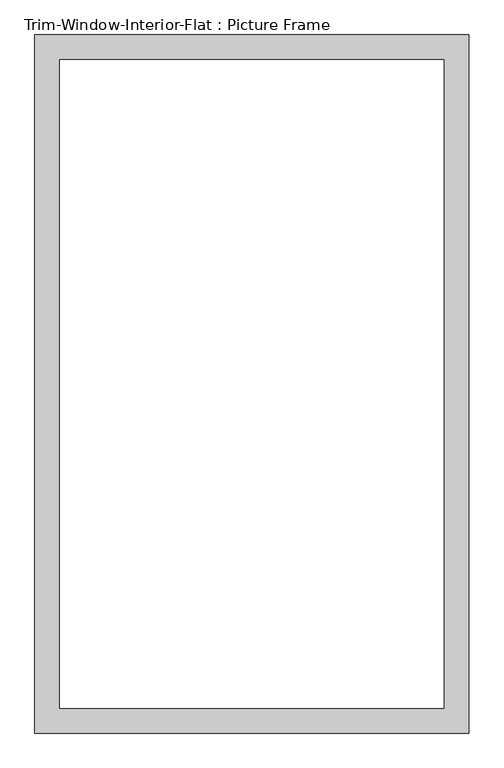
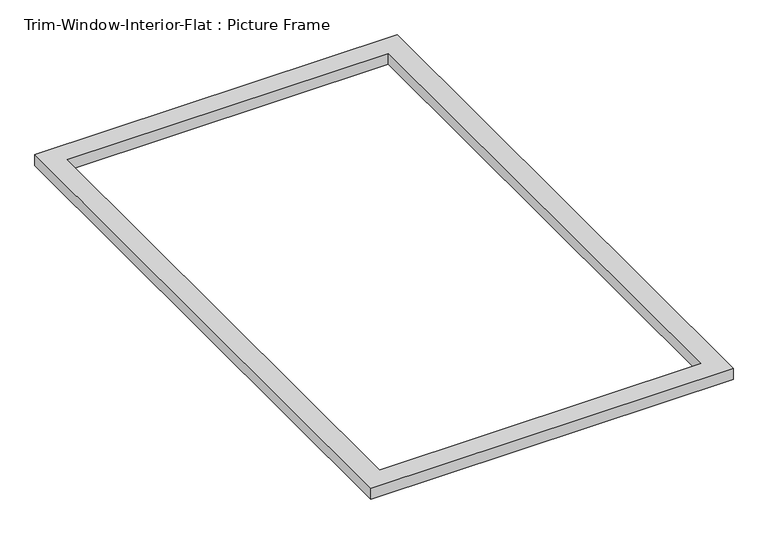
"""IFC4 building model written with IfcOpenShell, lengths in millimetres: proxy geometry, Trim-Window-Interior-Flat : Picture Frame."""

import ifcopenshell
import ifcopenshell.guid

model = None  # the IFC model being written
_history = None  # IfcOwnerHistory: only IFC2X3 demands one
_inside = {}  # id of a spatial element -> (the spatial element, [elements in it])
_under = {}  # id of a project, library or spatial element -> (it, [spatial elements below it])
_declared = {}  # id of a project -> (the project, [libraries it declares])
_typed = {}  # id of a type object -> (the type object, [elements of that type])
_made_of = {}  # id of a material, layer set ... -> (it, [elements and type objects made of it])


def new_model(schema):
    """Start an empty IFC model of exactly this schema.

    Asked for "IFC4X3", IfcOpenShell would pick the latest addendum, in which some entities
    have other attributes; the version numbers below select the first issue.
    IFC2X3 requires an IfcOwnerHistory on every rooted entity: one is made here for all.
    """
    global model, _history
    if schema == "IFC4X3":
        model = ifcopenshell.file(schema_version=(4, 3, 0, 0))
    else:
        model = ifcopenshell.file(schema=schema)
    _inside.clear()
    _under.clear()
    _declared.clear()
    _typed.clear()
    _made_of.clear()
    _history = None
    if model.schema == "IFC2X3":
        org = make("IfcOrganization", Name="unknown")
        user = make(
            "IfcPersonAndOrganization",
            ThePerson=make("IfcPerson", FamilyName="unknown"),
            TheOrganization=org,
        )
        app = make(
            "IfcApplication",
            ApplicationDeveloper=org,
            Version="unknown",
            ApplicationFullName="unknown",
            ApplicationIdentifier="unknown",
        )
        _history = make(
            "IfcOwnerHistory",
            OwningUser=user,
            OwningApplication=app,
            ChangeAction="ADDED",
            CreationDate=0,
        )
    return model


def make(cls, **values):
    """One entity of the class cls with the attributes given. An attribute that is None is left unset."""
    return model.create_entity(
        cls, **{name: value for name, value in values.items() if value is not None}
    )


def rooted(cls, **values):
    """An entity with a GlobalId (a new one), such as an element, a storey or a relation."""
    return make(cls, GlobalId=ifcopenshell.guid.new(), OwnerHistory=_history, **values)


def si_unit(unit_type, name, prefix=None):
    """IfcSIUnit, for example si_unit("LENGTHUNIT", "METRE", prefix="MILLI")."""
    return make("IfcSIUnit", UnitType=unit_type, Prefix=prefix, Name=name)


def assignment(units):
    """IfcUnitAssignment: the units of a project."""
    return None if units is None else make("IfcUnitAssignment", Units=units)


def point(xyz):
    """IfcCartesianPoint."""
    return None if xyz is None else make("IfcCartesianPoint", Coordinates=xyz)


def direction(xyz):
    """IfcDirection."""
    return None if xyz is None else make("IfcDirection", DirectionRatios=xyz)


def frame(location, z_axis=None, x_axis=None):
    """IfcAxis2Placement3D, a coordinate frame: its origin and axes. An axis left out is left unset."""
    return make(
        "IfcAxis2Placement3D",
        Location=point(location),
        Axis=direction(z_axis),
        RefDirection=direction(x_axis),
    )


def origin():
    """The frame at (0, 0, 0) with its axes left unset."""
    return frame((0.0, 0.0, 0.0))


def origin_with_axes():
    """The frame at (0, 0, 0) with the z axis (0, 0, 1) and the x axis (1, 0, 0) written out."""
    return frame((0.0, 0.0, 0.0), z_axis=(0.0, 0.0, 1.0), x_axis=(1.0, 0.0, 0.0))


def place(relative_to, where):
    """IfcLocalPlacement: puts the frame where relative to a parent placement (None: the world)."""
    return make(
        "IfcLocalPlacement", PlacementRelTo=relative_to, RelativePlacement=where
    )


def context(
    kind, dimensions, precision=None, world=None, true_north=None, identifier=None
):
    """IfcGeometricRepresentationContext, for example the 3D "Model" context."""
    return make(
        "IfcGeometricRepresentationContext",
        ContextIdentifier=identifier,
        ContextType=kind,
        CoordinateSpaceDimension=dimensions,
        Precision=precision,
        WorldCoordinateSystem=world,
        TrueNorth=true_north,
    )


def project(units=None, contexts=None):
    """IfcProject with its units and contexts."""
    return rooted(
        "IfcProject",
        Name="project",
        RepresentationContexts=contexts,
        UnitsInContext=assignment(units),
    )


def spatial(cls, under=None, at=None, **own):
    """A site, building, storey or space (cls), placed at a placement, below another one or the project."""
    s = rooted(cls, ObjectPlacement=at, **own)
    if under is not None:
        _under.setdefault(under.id(), (under, []))[1].append(s)
    return s


def polyline(points):
    """IfcPolyline through the points."""
    return make("IfcPolyline", Points=[point(p) for p in points])


def outline(outer, holes=None, kind="AREA"):
    """IfcArbitraryClosedProfileDef: a profile drawn as a closed curve; with holes, ...WithVoids."""
    if holes is None:
        return make("IfcArbitraryClosedProfileDef", ProfileType=kind, OuterCurve=outer)
    return make(
        "IfcArbitraryProfileDefWithVoids",
        ProfileType=kind,
        OuterCurve=outer,
        InnerCurves=holes,
    )


def extrude(swept, where, along, depth):
    """IfcExtrudedAreaSolid: the profile swept, set in the frame where, extruded along a direction by depth."""
    return make(
        "IfcExtrudedAreaSolid",
        SweptArea=swept,
        Position=where,
        ExtrudedDirection=direction(along),
        Depth=depth,
    )


def shape(context_of_items, identifier, shape_type, items):
    """IfcShapeRepresentation: the items that make up one representation, for example the "Body"."""
    return make(
        "IfcShapeRepresentation",
        ContextOfItems=context_of_items,
        RepresentationIdentifier=identifier,
        RepresentationType=shape_type,
        Items=items,
    )


def source(mapping_origin, context_of_items, identifier, shape_type, items):
    """IfcRepresentationMap: a shape defined once, which mapped items show again and again."""
    return make(
        "IfcRepresentationMap",
        MappingOrigin=mapping_origin,
        MappedRepresentation=shape(context_of_items, identifier, shape_type, items),
    )


def transform(
    local_origin,
    x_axis=None,
    y_axis=None,
    z_axis=None,
    scale=None,
    scale2=None,
    scale3=None,
    uniform=True,
):
    """IfcCartesianTransformationOperator3D, or its non-uniform kind. x_axis, y_axis, z_axis: its Axis1, 2, 3."""
    if uniform:
        return make(
            "IfcCartesianTransformationOperator3D",
            Axis1=direction(x_axis),
            Axis2=direction(y_axis),
            LocalOrigin=point(local_origin),
            Scale=scale,
            Axis3=direction(z_axis),
        )
    return make(
        "IfcCartesianTransformationOperator3DnonUniform",
        Axis1=direction(x_axis),
        Axis2=direction(y_axis),
        LocalOrigin=point(local_origin),
        Scale=scale,
        Axis3=direction(z_axis),
        Scale2=scale2,
        Scale3=scale3,
    )


def mapped(mapping_source, mapping_target):
    """IfcMappedItem: shows the shape of a source again, moved by a transform."""
    return make(
        "IfcMappedItem", MappingSource=mapping_source, MappingTarget=mapping_target
    )


def made_of(thing, what):
    """Note that an element or type object is made of a material, layer set ...; save() writes the relation."""
    if what is not None:
        _made_of.setdefault(what.id(), (what, []))[1].append(thing)
    return thing


def element(
    cls,
    number,
    at=None,
    inside=None,
    cuts=None,
    type_object=None,
    material=None,
    context=None,
    identifier="Body",
    shape_type=None,
    held_by="IfcProductDefinitionShape",
    body=None,
    shapes=None,
    **own,
):
    """One element of the class cls, such as IfcWall. Its Tag is "e" and its number.

    at: its placement. inside: the storey or other place that contains it. cuts: it is an
    opening in that element (IfcRelVoidsElement). A single representation is given by context,
    identifier, shape_type and body (its items); several are given by shapes. held_by: the class
    of the entity that holds the representations. save() writes the other relations.
    """
    e = rooted(cls, Tag="e%d" % number, ObjectPlacement=at, **own)
    if body is not None:
        shapes = [shape(context, identifier, shape_type, body)]
    if shapes is not None:
        e.Representation = make(held_by, Representations=shapes)
    if inside is not None:
        _inside.setdefault(inside.id(), (inside, []))[1].append(e)
    if cuts is not None:
        rooted(
            "IfcRelVoidsElement", RelatingBuildingElement=cuts, RelatedOpeningElement=e
        )
    if type_object is not None:
        _typed.setdefault(type_object.id(), (type_object, []))[1].append(e)
    return made_of(e, material)


def aggregate(whole, parts):
    """IfcRelAggregates: a whole, such as a stair, and the parts it consists of."""
    return rooted("IfcRelAggregates", RelatingObject=whole, RelatedObjects=parts)


def save(model, path):
    """Write the relations noted so far, then the file.

    IfcRelAggregates (storeys below a building ...), IfcRelContainedInSpatialStructure (elements
    in a storey), IfcRelDefinesByType, IfcRelAssociatesMaterial and IfcRelDeclares: one each for
    every whole, place, type object, material and project.
    """
    for whole, parts in _under.values():
        aggregate(whole, parts)
    for where, things in _inside.values():
        rooted(
            "IfcRelContainedInSpatialStructure",
            RelatedElements=things,
            RelatingStructure=where,
        )
    for kind, things in _typed.values():
        rooted("IfcRelDefinesByType", RelatedObjects=things, RelatingType=kind)
    for what, things in _made_of.values():
        rooted("IfcRelAssociatesMaterial", RelatedObjects=things, RelatingMaterial=what)
    for by, libraries in _declared.values():
        rooted("IfcRelDeclares", RelatingContext=by, RelatedDefinitions=libraries)
    model.write(path)


def trim_window_interior_flat_picture_frame_3667116f(model_context):
    return source(origin(), model_context, "Body", "SweptSolid", [
        extrude(outline(polyline([(501.65, 44.45), (501.65, -1568.45), (-501.65, -1568.45), (-501.65, 44.45), (501.65, 44.45)]), holes=[polyline([(444.5, -12.7), (-444.5, -12.7), (-444.5, -1511.3), (444.5, -1511.3), (444.5, -12.7)])]), origin_with_axes(), (0.0, 0.0, 1.0), 31.75),
    ])


if __name__ == "__main__":
    model = new_model("IFC4")
    model_context = context("Model", 3, world=origin())
    ifc_project = project(units=[si_unit("LENGTHUNIT", "METRE", prefix="MILLI")], contexts=[model_context])
    site = spatial("IfcSite", under=ifc_project)
    building = spatial("IfcBuilding", under=site)
    placement = place(None, origin())
    trim_window_interior_flat_picture_frame_shape = trim_window_interior_flat_picture_frame_3667116f(model_context)
    element("IfcBuildingElementProxy", 1, Name="Trim-Window-Interior-Flat : Picture Frame", ObjectType="Trim-Window-Interior-Flat : Picture Frame", at=placement, inside=building, context=model_context, shape_type="MappedRepresentation", body=[
        mapped(trim_window_interior_flat_picture_frame_shape, transform((0.0, 0.0, 0.0), x_axis=(1.0, 0.0, 0.0), y_axis=(0.0, 1.0, 0.0), z_axis=(0.0, 0.0, 1.0))),
    ])
    save(model, "model.ifc")

# Revit data of these elements
# Type "Trim-Window-Interior-Flat : Picture Frame"
#   Trim Thickness_Picture Frame = 0' - 1 1/4"
#   Trim Width = 0' - 2 1/4"
#   Trim Thickness_with Sill = 0' - 0 3/4"
#   Sill Thickness = 0' - 1 1/4"
#   Opening Width [instance default] = 2' - 0"
#   Opening Height [instance default] = 3' - 0"
#   Default Elevation = 4' - 0"
#   Sill = no
#   Picture Frame = yes
#   Trim Material [instance default] = none
# Element 1 (IfcBuildingElementProxy, "Trim-Window-Interior-Flat : Picture Frame")
#   Opening Width = 3' - 0"
#   Opening Height = 5' - 0"
#   Trim Material = Wood - Stained
#   Materials on its faces: "Wood - Stained"
# Materials
#   "Wood - Stained": class "Wood", colour RGB 224 178 126, transparency 0, Cost = 0
